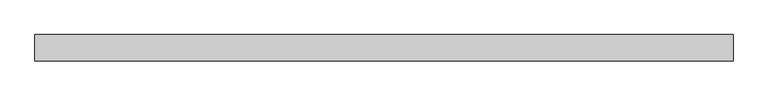
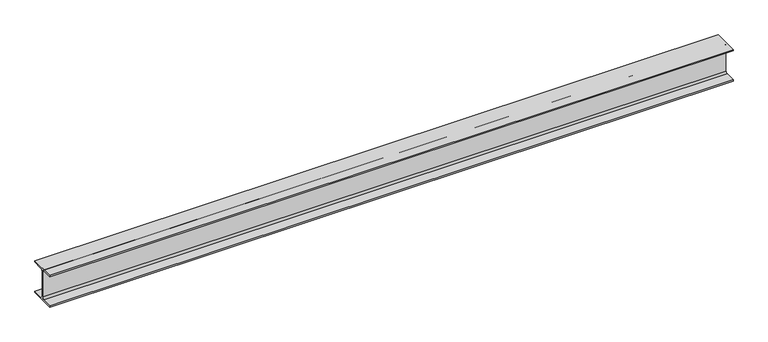
"""IFC4 building model written with IfcOpenShell, lengths in millimetres: beam geometry, 0912_Steel Framing_H-KSD3502 : H_SB_ASB_H-390x300x10x16."""

from ifc_helpers import new_model, si_unit, point, frame, frame_2d, origin, place, context, project, spatial, polyline, circle_curve, trimmed, segment, composite_curve, outline, extrude, source, transform, mapped, element, save


def beam_8a1f8e14(model_context):
    return source(origin(), model_context, "Body", "SweptSolid", [
        extrude(outline(composite_curve([segment(polyline([(150.0, -179.0), (150.0, -195.0), (-150.0, -195.0), (-150.0, -179.0), (-27.0, -179.0)]), True, "CONTINUOUS"), segment(trimmed(circle_curve(frame_2d((-27.0, -157.0)), 22.0), [point((-27.0, -179.0))], [point((-5.0, -157.0))], True, "CARTESIAN"), True, "CONTINUOUS"), segment(polyline([(-5.0, -157.0), (-5.0, 157.0)]), True, "CONTINUOUS"), segment(trimmed(circle_curve(frame_2d((-27.0, 157.0)), 22.0), [point((-5.0, 157.0))], [point((-27.0, 179.0))], True, "CARTESIAN"), True, "CONTINUOUS"), segment(polyline([(-27.0, 179.0), (-150.0, 179.0), (-150.0, 195.0), (150.0, 195.0), (150.0, 179.0), (27.0, 179.0)]), True, "CONTINUOUS"), segment(trimmed(circle_curve(frame_2d((27.0, 157.0)), 22.0), [point((27.0, 179.0))], [point((5.0, 157.0))], True, "CARTESIAN"), True, "CONTINUOUS"), segment(polyline([(5.0, 157.0), (5.0, -157.0)]), True, "CONTINUOUS"), segment(trimmed(circle_curve(frame_2d((27.0, -157.0)), 22.0), [point((5.0, -157.0))], [point((27.0, -179.0))], True, "CARTESIAN"), True, "CONTINUOUS"), segment(polyline([(27.0, -179.0), (150.0, -179.0)]), True, "CONTINUOUS")], self_intersect=False)), frame((-3987.2999994, 0.0, 0.0), z_axis=(1.0, 0.0, 0.0), x_axis=(0.0, 1.0, 0.0)), (0.0, 0.0, 1.0), 7974.5999988),
    ])


if __name__ == "__main__":
    model = new_model("IFC4")
    model_context = context("Model", 3, world=origin())
    ifc_project = project(units=[si_unit("LENGTHUNIT", "METRE", prefix="MILLI")], contexts=[model_context])
    site = spatial("IfcSite", under=ifc_project)
    building = spatial("IfcBuilding", under=site)
    placement = place(None, origin())
    beam_shape = beam_8a1f8e14(model_context)
    element("IfcBeam", 1, ObjectType="0912_Steel Framing_H-KSD3502 : H_SB_ASB_H-390x300x10x16", at=placement, inside=building, context=model_context, shape_type="MappedRepresentation", body=[
        mapped(beam_shape, transform((0.0, 0.0, 0.0), x_axis=(1.0, 0.0, 0.0), y_axis=(0.0, 1.0, 0.0), z_axis=(0.0, 0.0, 1.0))),
    ])
    save(model, "model.ifc")

# Revit data of these elements
# Type "0912_Steel Framing_H-KSD3502 : H_SB_ASB_H-390x300x10x16"
#   H_WM Code_1 = "S01AA001-00001 | Main Steel Structure Fabrication Work | Shelter/Building | Heavy Steel - Standard (Weight≥90KG/M) | Material: (   )"
#   H_WM Code_2 = "S03AA027-00001 | Main Steel Structure Erection Work | Shelter/Building | Heavy Steel (Weight≥90KG/M) | Material: (   )"
#   H_WM Code_3 = "S01AA010-00001 | Main Steel Structure Fabrication Work | Shelter/Building | Steel Painting/Coating | for Non-Fireproofed Steel Surface, Surface Preparation, Primer, Second & Final Coat | Material: (   )"
#   H_Q'ty Cal Type Tag = "SB-Q2"
#   Width = 30.0 cm
#   Web Thickness = 1.0 cm
#   Web Fillet = 2.2 cm
#   Warping Constant = 2520000.0 cm⁶
#   W = 0
#   Torsional Moment of Inertia = 94.3867 cm⁴
#   Section Area = 136.0 cm²
#   Plastic Modulus weak axis = 733.0 cm³
#   Plastic Modulus strong axis = 2190.0 cm³
#   Perimeter = 1.92 m²/m
#   Nominal Weight = 107.00 kgf/m
#   Moment of Inertia weak axis = 7210.00 cm⁴
#   Moment of Inertia strong axis = 38700.00 cm⁴
#   Height = 39.0 cm
#   Flange Thickness = 1.6 cm
#   Elastic Modulus weak axis = 481.0 cm³
#   Elastic Modulus strong axis = 1980.0 cm³
#   Centroid Vertical = 19.5 cm
#   Centroid Horizontal = 15.0 cm
#   Ix = 387000000
#   Length [instance default] = 1.5240 m
#   Zx = 2190000
#   b = 0.3000 m
#   h = 0.3900 m
#   r = 0.0220 m
#   s = 0.0100 m
#   t = 0.0160 m
#   A = 0.0136 m²
#   Structural Material [instance default] = Steel, 45-345
#   Assembly Code = ""
# Element 1 (IfcBeam, "0912_Steel Framing_H-KSD3502 : H_SB_ASB_H-390x300x10x16")
#   Structural Material = none
# Materials
#   "Steel, 45-345": class "Metal", colour RGB 189 187 185, transparency 0, Description = "Steel 345 MPa", Cost = 0
